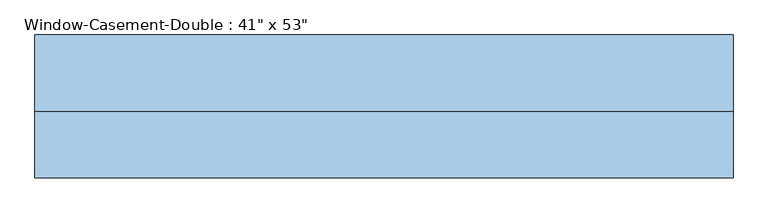
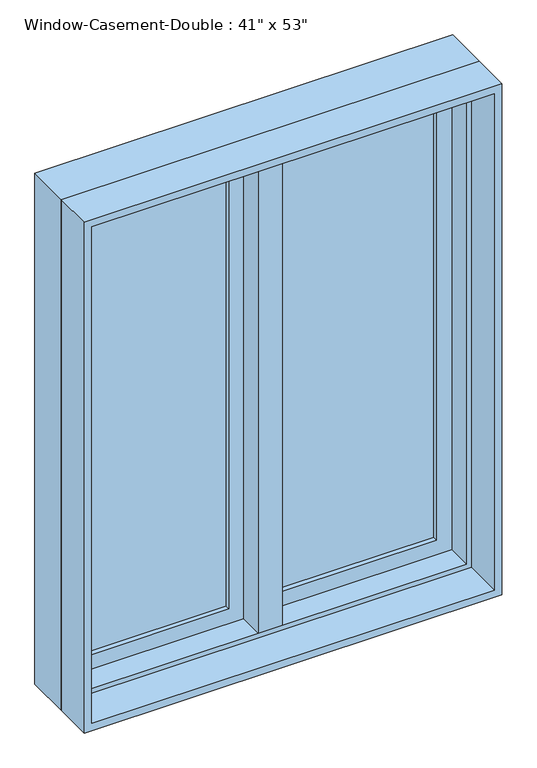
"""IFC4 building model written with IfcOpenShell, lengths in millimetres: window geometry."""

from ifc_helpers import new_model, si_unit, frame, origin, place, context, project, spatial, polyline, outline, extrude, faceted_brep, source, transform, mapped, element, save


def window_fe860c6c(model_context):
    return source(origin(), model_context, "Body", "SolidModel", [
        faceted_brep([(9.525, 115.8875, 2247.9), (-9.525, 115.8875, 2247.9), (-9.525, 65.0875, 2247.9), (9.525, 65.0875, 2247.9), (9.525, 115.8875, 927.1), (9.525, 65.0875, 927.1), (-9.525, 65.0875, 927.1), (-9.525, 115.8875, 927.1), (-9.525, 65.0875, 946.15), (-9.525, 65.0875, 2228.85), (-30.1625, 65.0875, 946.15), (-30.1625, 65.0875, 2228.85), (-30.1625, 1.5875, 946.15), (-30.1625, 1.5875, 2228.85), (30.1625, 1.5875, 946.15), (30.1625, 1.5875, 2228.85), (30.1625, 65.0875, 946.15), (30.1625, 65.0875, 2228.85), (9.525, 65.0875, 946.15), (9.525, 65.0875, 2228.85)], [[[0, 1, 2, 3]], [[4, 5, 6, 7]], [[1, 0, 4, 7]], [[2, 1, 7, 6, 8, 9]], [[9, 8, 10, 11]], [[11, 10, 12, 13]], [[13, 12, 14, 15]], [[15, 14, 16, 17]], [[17, 16, 18, 19]], [[0, 3, 19, 18, 5, 4]], [[18, 8, 6, 5]], [[9, 19, 3, 2]], [[8, 18, 16, 14, 12, 10]], [[19, 9, 11, 13, 15, 17]]]),
        extrude(outline(polyline([(-66.675, 96.8375), (-66.675, 90.4875), (-450.85, 90.4875), (-450.85, 96.8375), (-66.675, 96.8375)])), frame((0.0, 0.0, 984.25), z_axis=(0.0, 0.0, 1.0), x_axis=(1.0, 0.0, 0.0)), (0.0, 0.0, 1.0), 1206.5),
        extrude(outline(polyline([(-450.85, 77.7875), (-450.85, 84.1375), (-66.675, 84.1375), (-66.675, 77.7875), (-450.85, 77.7875)])), frame((0.0, 0.0, 984.25), z_axis=(0.0, 0.0, 1.0), x_axis=(1.0, 0.0, 0.0)), (0.0, 0.0, 1.0), 1206.5),
        extrude(outline(polyline([(450.85, 96.8375), (450.85, 90.4875), (66.675, 90.4875), (66.675, 96.8375), (450.85, 96.8375)])), frame((0.0, 0.0, 984.25), z_axis=(0.0, 0.0, 1.0), x_axis=(1.0, 0.0, 0.0)), (0.0, 0.0, 1.0), 1206.5),
        extrude(outline(polyline([(66.675, 77.7875), (66.675, 84.1375), (450.85, 84.1375), (450.85, 77.7875), (66.675, 77.7875)])), frame((0.0, 0.0, 984.25), z_axis=(0.0, 0.0, 1.0), x_axis=(1.0, 0.0, 0.0)), (0.0, 0.0, 1.0), 1206.5),
        extrude(outline(polyline([(2247.9, -508.0), (927.1, -508.0), (927.1, -9.525), (2247.9, -9.525), (2247.9, -508.0)]), holes=[polyline([(2190.75, -66.675), (984.25, -66.675), (984.25, -450.85), (2190.75, -450.85), (2190.75, -66.675)])]), frame((0.0, 65.0875, 0.0), z_axis=(0.0, 1.0, 0.0), x_axis=(0.0, 0.0, 1.0)), (0.0, 0.0, 1.0), 44.45),
        extrude(outline(polyline([(927.1, 508.0), (2247.9, 508.0), (2247.9, 9.525), (927.1, 9.525), (927.1, 508.0)]), holes=[polyline([(984.25, 66.675), (2190.75, 66.675), (2190.75, 450.85), (984.25, 450.85), (984.25, 66.675)])]), frame((0.0, 65.0875, 0.0), z_axis=(0.0, 1.0, 0.0), x_axis=(0.0, 0.0, 1.0)), (0.0, 0.0, 1.0), 44.45),
        extrude(outline(polyline([(2260.6, -520.7), (914.4, -520.7), (914.4, 520.7), (2260.6, 520.7), (2260.6, -520.7)]), holes=[polyline([(2241.55, 501.65), (933.45, 501.65), (933.45, -501.65), (2241.55, -501.65), (2241.55, 501.65)])]), frame((0.0, -96.8375, 0.0), z_axis=(0.0, 1.0, 0.0), x_axis=(0.0, 0.0, 1.0)), (0.0, 0.0, 1.0), 98.425),
        faceted_brep([(488.95, 65.0875, 2228.85), (488.95, 1.5875, 2228.85), (-488.95, 1.5875, 2228.85), (-488.95, 65.0875, 2228.85), (508.0, 115.8875, 2247.9), (508.0, 65.0875, 2247.9), (-508.0, 65.0875, 2247.9), (-508.0, 115.8875, 2247.9), (520.7, 1.5875, 2260.6), (520.7, 115.8875, 2260.6), (-520.7, 115.8875, 2260.6), (-520.7, 1.5875, 2260.6), (-488.95, 1.5875, 946.15), (-488.95, 65.0875, 946.15), (-508.0, 65.0875, 927.1), (-508.0, 115.8875, 927.1), (-520.7, 115.8875, 914.4), (-520.7, 1.5875, 914.4), (488.95, 1.5875, 946.15), (488.95, 65.0875, 946.15), (508.0, 65.0875, 927.1), (508.0, 115.8875, 927.1), (520.7, 115.8875, 914.4), (520.7, 1.5875, 914.4)], [[[0, 1, 2, 3]], [[4, 5, 6, 7]], [[8, 9, 10, 11]], [[3, 2, 12, 13]], [[7, 6, 14, 15]], [[11, 10, 16, 17]], [[13, 12, 18, 19]], [[15, 14, 20, 21]], [[17, 16, 22, 23]], [[11, 17, 23, 8], [1, 18, 12, 2]], [[19, 18, 1, 0]], [[5, 20, 14, 6], [3, 13, 19, 0]], [[21, 20, 5, 4]], [[23, 22, 9, 8]], [[9, 22, 16, 10], [7, 15, 21, 4]]]),
    ])


if __name__ == "__main__":
    model = new_model("IFC4")
    model_context = context("Model", 3, world=origin())
    ifc_project = project(units=[si_unit("LENGTHUNIT", "METRE", prefix="MILLI")], contexts=[model_context])
    site = spatial("IfcSite", under=ifc_project)
    building = spatial("IfcBuilding", under=site)
    placement = place(None, origin())
    window_shape = window_fe860c6c(model_context)
    element("IfcWindow", 1, ObjectType="Window-Casement-Double : 41\" x 53\"", at=placement, inside=building, context=model_context, shape_type="MappedRepresentation", body=[
        mapped(window_shape, transform((0.0, 0.0, 0.0), x_axis=(1.0, 0.0, 0.0), y_axis=(0.0, 1.0, 0.0), z_axis=(0.0, 0.0, 1.0))),
    ])
    save(model, "model.ifc")

# Revit data of these elements
# Type "Window-Casement-Double : 41\" x 53\""
#   Type Mark = "60"
#   Fire Rating = "0.5h"
#   Assembly Code = "B2020100"
#   Analytic Construction = "Double glazing - domestic"
#   Frame Extension [instance default] = 0' - 0 1/4"
#   Window Inset [instance default] = 0' - 0"
#   Wall Thickness [instance default] = 0' - 6"
#   Interior Wall Closure [instance default] = 0' - 2 1/4"
#   Half Width = 1' - 8 1/2"
#   Visual Light Transmittance = 0.81
#   Thermal Resistance (R) = 1.8146 (h·ft²·°F)/BTU
#   Solar Heat Gain Coefficient = 0.76
#   Rough Width = 3' - 5 1/2"
#   Rough Height = 4' - 5 1/2"
#   Height = 4' - 5"
#   Heat Transfer Coefficient (U) = 0.5511 BTU/(h·ft²·°F)
#   Exterior Wall Closure [instance default] = 0' - 1 1/4"
#   Extension Jamb [instance default] = 0' - 2 1/4"
#   Default Sill Height = 3' - 0"
#   Width = 3' - 5"
#   Define Thermal Properties by = 0
#   Muntin Visibility = yes
#   Interior Trim Visibility [instance default] = yes
#   Exterior Trim Visibility [instance default] = yes
#   Extension Jamb Visibility [instance default] = yes
#   Interior Trim Material = Wood - Stained
#   Muntin Pattern = Muntin Pattern_2x2 : Muntin Pattern_2x2
#   Interior Trim = Trim-Window-Interior-Flat : Picture Frame
#   Interior Frame Material = Wood - Stained
#   Glass Panel Material = Glass
#   Exterior Trim Material = Clad - White
#   Exterior Trim = Trim-Window-Exterior-Flat : with Sill
#   Exterior Frame Material = Clad - White
#   Wall Closure = (empty or 0)
# Element 1 (IfcWindow, "Window-Casement-Double : 41\" x 53\"")
#   Wall Thickness = 0' - 7 5/8"
#   Extension Jamb = 0' - 3 7/8"
#   Materials on its faces: "Wood - Stained", "Glass", "Clad - White"
# Materials
#   "Wood - Stained": class "Wood", colour RGB 224 178 126, transparency 0, Cost = 0
#   "Glass": class "Glass", colour RGB 236 240 239, transparency 0.5, Description = "Soda Lime Glass", Cost = 0
#   "Clad - White": class "Wood", colour RGB 216 216 204, transparency 0, Cost = 0
